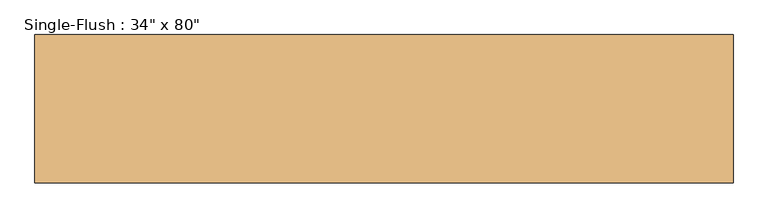
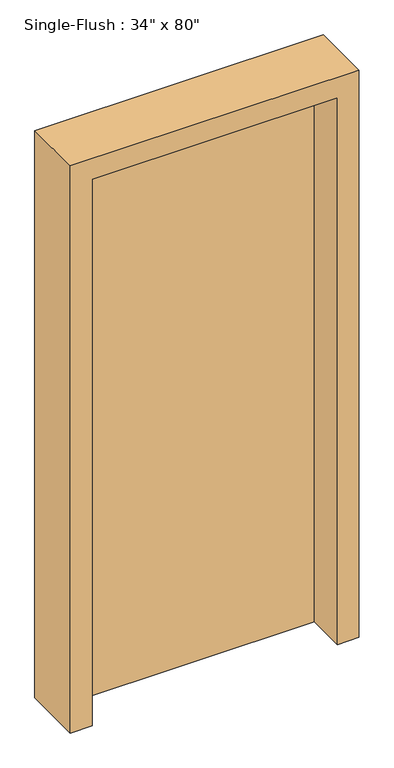
"""IFC4 building model written with IfcOpenShell, lengths in millimetres: door geometry."""

from ifc_helpers import new_model, si_unit, frame, origin, origin_with_axes, place, context, project, spatial, polyline, outline, extrude, source, transform, mapped, element, save


def door_46dfc76b(model_context):
    return source(origin(), model_context, "Body", "SweptSolid", [
        extrude(outline(polyline([(2108.2, 508.0), (2108.2, -508.0), (0.0, -508.0), (0.0, -431.8), (2032.0, -431.8), (2032.0, 431.8), (0.0, 431.8), (0.0, 508.0), (2108.2, 508.0)])), frame((0.0, -107.95, 0.0), z_axis=(0.0, 1.0, 0.0), x_axis=(0.0, 0.0, 1.0)), (0.0, 0.0, 1.0), 215.9),
        extrude(outline(polyline([(431.8, 31.75), (-431.8, 31.75), (-431.8, 82.55), (431.8, 82.55), (431.8, 31.75)])), origin_with_axes(), (0.0, 0.0, 1.0), 2032.0),
    ])


if __name__ == "__main__":
    model = new_model("IFC4")
    model_context = context("Model", 3, world=origin())
    ifc_project = project(units=[si_unit("LENGTHUNIT", "METRE", prefix="MILLI")], contexts=[model_context])
    site = spatial("IfcSite", under=ifc_project)
    building = spatial("IfcBuilding", under=site)
    placement = place(None, origin())
    door_shape = door_46dfc76b(model_context)
    element("IfcDoor", 1, ObjectType="Single-Flush : 34\" x 80\"", at=placement, inside=building, context=model_context, shape_type="MappedRepresentation", body=[
        mapped(door_shape, transform((0.0, 0.0, 0.0), x_axis=(1.0, 0.0, 0.0), y_axis=(0.0, 1.0, 0.0), z_axis=(0.0, 0.0, 1.0))),
    ])
    save(model, "model.ifc")

# Revit data of these elements
# Type "Single-Flush : 34\" x 80\""
#   Type Mark = "7"
#   OD_DS_Door_Material = "T.B.D."
#   OD_DS_Door_Type = "SWING"
#   OD_DS_Lockset = "PRIVACY LOCK"
#   Assembly Code = "C1020"
#   Analytic Construction = "<None>"
#   Thickness = 0' - 2"
#   RO Offset = 0' - 0 1/4"
#   Height = 6' - 8"
#   Trim Projection Ext = 0' - 1"
#   Trim Projection Int = 0' - 1"
#   Trim Width = 0' - 3"
#   Width = 2' - 10"
#   Door Material = Closet_1
#   Frame Material = Closet_1
#   Function = (empty or 0)
#   Wall Closure = (empty or 0)
# Element 1 (IfcDoor, "Single-Flush : 34\" x 80\"")
#   Materials on its faces: "Closet_1"
# Materials
#   "Closet_1": class "Paint", colour RGB 200 194 183, transparency 0, Cost = 0
